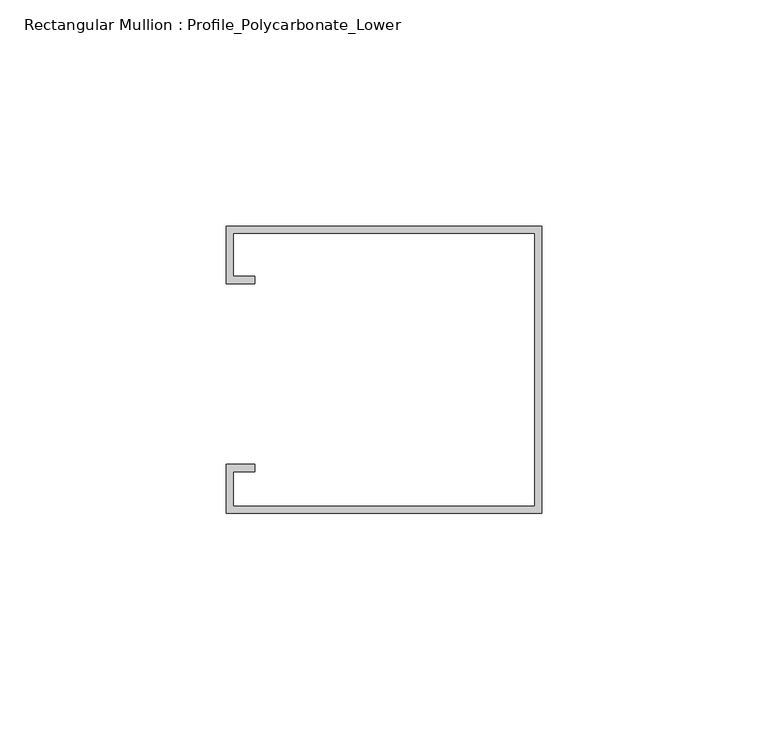
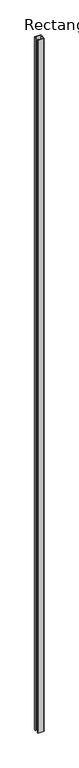
"""IFC4 building model written with IfcOpenShell, lengths in millimetres: member geometry, Rectangular Mullion : Profile_Polycarbonate_Lower."""

from ifc_helpers import new_model, si_unit, frame, origin, place, context, project, spatial, polyline, outline, extrude, source, transform, mapped, element, save


def rectangular_mullion_profile_polycarbonate_lower_4e553c8f(model_context):
    return source(origin(), model_context, "Body", "SweptSolid", [
        extrude(outline(polyline([(0.0, 32.7), (0.0, -30.8), (-69.85, -30.8), (-69.85, -20.0), (-63.5, -20.0), (-63.5, -21.5875), (-68.2625, -21.5875), (-68.2625, -29.2125), (-1.5875, -29.2125), (-1.5875, 31.1125), (-68.2625, 31.1125), (-68.2625, 21.5875), (-63.5, 21.5875), (-63.5, 20.0), (-69.85, 20.0), (-69.85, 32.7), (0.0, 32.7)])), frame((0.0, 0.0, -8370.8875), z_axis=(0.0, 0.0, 1.0), x_axis=(1.0, 0.0, 0.0)), (0.0, 0.0, 1.0), 8370.8875),
    ])


if __name__ == "__main__":
    model = new_model("IFC4")
    model_context = context("Model", 3, world=origin())
    ifc_project = project(units=[si_unit("LENGTHUNIT", "METRE", prefix="MILLI")], contexts=[model_context])
    site = spatial("IfcSite", under=ifc_project)
    building = spatial("IfcBuilding", under=site)
    placement = place(None, origin())
    rectangular_mullion_profile_polycarbonate_lower_shape = rectangular_mullion_profile_polycarbonate_lower_4e553c8f(model_context)
    element("IfcMember", 1, ObjectType="Rectangular Mullion : Profile_Polycarbonate_Lower", at=placement, inside=building, context=model_context, shape_type="MappedRepresentation", body=[
        mapped(rectangular_mullion_profile_polycarbonate_lower_shape, transform((0.0, 0.0, 0.0), x_axis=(1.0, 0.0, 0.0), y_axis=(0.0, 1.0, 0.0), z_axis=(0.0, 0.0, 1.0))),
    ])
    save(model, "model.ifc")

# Revit data of these elements
# Type "Rectangular Mullion : Profile_Polycarbonate_Lower"
#   built-in parameter 1007322 = 0.208333 (stored number, unit not read)
#   built-in parameter 1007321 = 0 (stored number, unit not read)
#   built-in parameter 1007320 = 0.00520833 (stored number, unit not read)
